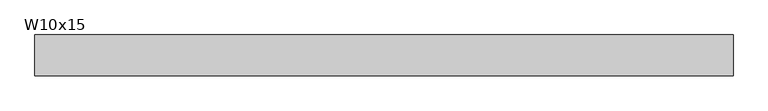
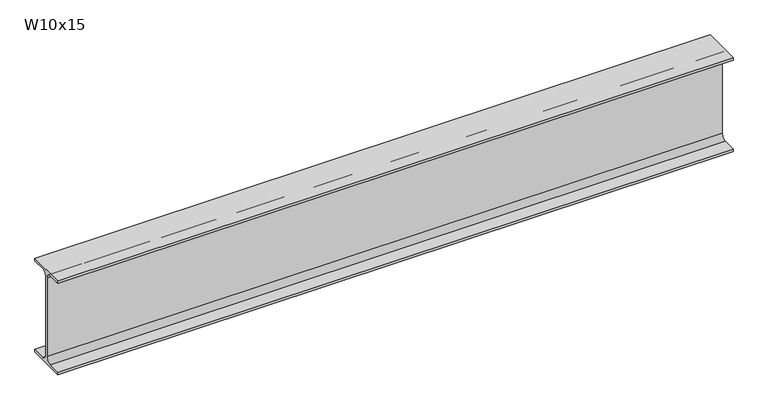
"""IFC4 building model written with IfcOpenShell, lengths in millimetres: beam geometry, RME W-Wide Flange : W10x15."""

from ifc_helpers import new_model, si_unit, point, frame, frame_2d, origin, place, context, project, spatial, polyline, circle_curve, trimmed, segment, composite_curve, outline, extrude, source, transform, mapped, element, save


def w10x15_4d7435c7(model_context):
    return source(origin(), model_context, "Body", "SweptSolid", [
        extrude(outline(composite_curve([segment(polyline([(50.8, -120.142), (50.8, -127.0), (-50.8, -127.0), (-50.8, -120.142), (-16.7005, -120.142)]), True, "CONTINUOUS"), segment(trimmed(circle_curve(frame_2d((-16.7005, -106.3625)), 13.7795), [point((-16.7005, -120.142))], [point((-2.921, -106.3625))], True, "CARTESIAN"), True, "CONTINUOUS"), segment(polyline([(-2.921, -106.3625), (-2.921, 106.3625)]), True, "CONTINUOUS"), segment(trimmed(circle_curve(frame_2d((-16.7005, 106.3625)), 13.7795), [point((-2.921, 106.3625))], [point((-16.7005, 120.142))], True, "CARTESIAN"), True, "CONTINUOUS"), segment(polyline([(-16.7005, 120.142), (-50.8, 120.142), (-50.8, 127.0), (50.8, 127.0), (50.8, 120.142), (16.7005, 120.142)]), True, "CONTINUOUS"), segment(trimmed(circle_curve(frame_2d((16.7005, 106.3625)), 13.7795), [point((16.7005, 120.142))], [point((2.921, 106.3625))], True, "CARTESIAN"), True, "CONTINUOUS"), segment(polyline([(2.921, 106.3625), (2.921, -106.3625)]), True, "CONTINUOUS"), segment(trimmed(circle_curve(frame_2d((16.7005, -106.3625)), 13.7795), [point((2.921, -106.3625))], [point((16.7005, -120.142))], True, "CARTESIAN"), True, "CONTINUOUS"), segment(polyline([(16.7005, -120.142), (50.8, -120.142)]), True, "CONTINUOUS")], self_intersect=False)), frame((-879.475, 0.0, 0.0), z_axis=(1.0, 0.0, 0.0), x_axis=(0.0, 1.0, 0.0)), (0.0, 0.0, 1.0), 1727.2),
    ])


if __name__ == "__main__":
    model = new_model("IFC4")
    model_context = context("Model", 3, world=origin())
    ifc_project = project(units=[si_unit("LENGTHUNIT", "METRE", prefix="MILLI")], contexts=[model_context])
    site = spatial("IfcSite", under=ifc_project)
    building = spatial("IfcBuilding", under=site)
    placement = place(None, origin())
    w10x15_shape = w10x15_4d7435c7(model_context)
    element("IfcBeam", 1, ObjectType="RME W-Wide Flange : W10x15", at=placement, inside=building, context=model_context, shape_type="MappedRepresentation", body=[
        mapped(w10x15_shape, transform((0.0, 0.0, 0.0), x_axis=(1.0, 0.0, 0.0), y_axis=(0.0, 1.0, 0.0), z_axis=(0.0, 0.0, 1.0))),
    ])
    save(model, "model.ifc")

# Revit data of these elements
# Type "RME W-Wide Flange : W10x15"
#   WELD P [instance default] = ""
#   WELD LE [instance default] = ""
#   WELD D [instance default] = ""
#   TOP SECTION SIZE [instance default] = ""
#   TOP SECTION LENGTH [instance default] = ""
#   REMARKS [instance default] = ""
#   REINF TYPE [instance default] = ""
#   Nominal Size = "W24"
#   End Bearing Capacity [instance default] = ""
#   BOT SECTION SIZE [instance default] = ""
#   BOT SECTION LENGTH [instance default] = ""
#   Assembly Code = "B10"
#   W = 15
#   Start Extension Calculation [instance default] = 10' - 0"
#   Start Extension [instance default] = -0' - 0 1/2"
#   End Extension Calculation [instance default] = 10' - 0"
#   End Extension [instance default] = -0' - 0 1/2"
#   Length [instance default] = 5' - 0"
#   bf = 0' - 4"
#   d = 0' - 10"
#   k = 0' - 0 13/16"
#   k2 = 0' - 0.5425"
#   tf = 0' - 0.27"
#   tw = 0' - 0.23"
#   A = 0.030625 SF
#   Structural Material [instance default] = Metal - Steel - ASTM A992
# Element 1 (IfcBeam, "RME W-Wide Flange : W10x15")
#   Length = 6' - 2 1/4"
#   Materials on its faces: "Metal - Steel - ASTM A992"
# Materials
#   "Metal - Steel - ASTM A992": class "Metal", colour RGB 255 128 0, transparency 0
